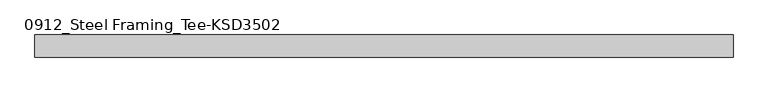
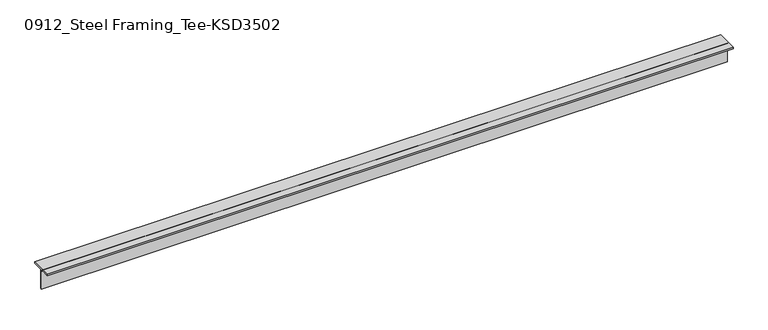
"""IFC4 building model written with IfcOpenShell, lengths in millimetres: member geometry, 0912_Steel Framing_Tee-KSD3502 : H_SB_ASB_CT-150x150x6.5x9."""

from ifc_helpers import new_model, si_unit, point, frame, frame_2d, origin, place, context, project, spatial, polyline, circle_curve, trimmed, segment, composite_curve, outline, extrude, source, transform, mapped, element, save


def member_0912_steel_framing_tee_ksd3502_f996880d(model_context):
    return source(origin(), model_context, "Body", "SweptSolid", [
        extrude(outline(composite_curve([segment(polyline([(-75.0, 75.0), (75.0, 75.0), (75.0, 66.0), (16.25, 66.0)]), True, "CONTINUOUS"), segment(trimmed(circle_curve(frame_2d((16.25, 53.0)), 13.0), [point((16.25, 66.0))], [point((3.25, 53.0))], True, "CARTESIAN"), True, "CONTINUOUS"), segment(polyline([(3.25, 53.0), (3.25, -75.0), (-3.25, -75.0), (-3.25, 53.0)]), True, "CONTINUOUS"), segment(trimmed(circle_curve(frame_2d((-16.25, 53.0)), 13.0), [point((-3.25, 53.0))], [point((-16.25, 66.0))], True, "CARTESIAN"), True, "CONTINUOUS"), segment(polyline([(-16.25, 66.0), (-75.0, 66.0), (-75.0, 75.0)]), True, "CONTINUOUS")], self_intersect=False)), frame((-2315.0, 0.0, 0.0), z_axis=(1.0, 0.0, 0.0), x_axis=(0.0, 1.0, 0.0)), (0.0, 0.0, 1.0), 4728.1),
    ])


if __name__ == "__main__":
    model = new_model("IFC4")
    model_context = context("Model", 3, world=origin())
    ifc_project = project(units=[si_unit("LENGTHUNIT", "METRE", prefix="MILLI")], contexts=[model_context])
    site = spatial("IfcSite", under=ifc_project)
    building = spatial("IfcBuilding", under=site)
    placement = place(None, origin())
    member_0912_steel_framing_tee_ksd3502_shape = member_0912_steel_framing_tee_ksd3502_f996880d(model_context)
    element("IfcMember", 1, ObjectType="0912_Steel Framing_Tee-KSD3502 : H_SB_ASB_CT-150x150x6.5x9", at=placement, inside=building, context=model_context, shape_type="MappedRepresentation", body=[
        mapped(member_0912_steel_framing_tee_ksd3502_shape, transform((0.0, 0.0, 0.0), x_axis=(1.0, 0.0, 0.0), y_axis=(0.0, 1.0, 0.0), z_axis=(0.0, 0.0, 1.0))),
    ])
    save(model, "model.ifc")

# Revit data of these elements
# Type "0912_Steel Framing_Tee-KSD3502 : H_SB_ASB_CT-150x150x6.5x9"
#   H_WM Code_1 = "S01AA003-00001 | Main Steel Structure Fabrication Work | Shelter/Building | Light Steel - Standard (30KG/M>Weight) | Material: (   )"
#   H_WM Code_2 = "S03AA029-00001 | Main Steel Structure Erection Work | Shelter/Building | Light Steel (30KG/M>Weight) | Material: (   )"
#   H_WM Code_3 = "S01AA010-00001 | Main Steel Structure Fabrication Work | Shelter/Building | Steel Painting/Coating | for Non-Fireproofed Steel Surface, Surface Preparation, Primer, Second & Final Coat | Material: (   )"
#   H_Q'ty Cal Type Tag = "SB-Q2"
#   Width = 15.0 cm
#   Web Thickness = 0.65 cm
#   Web Fillet = 1.3 cm
#   Section Area = 23.39 cm²
#   Perimeter = 0.60 m²/m
#   Nominal Weight = 18.40 kgf/m
#   Height = 15.0 cm
#   Flange Thickness = 0.9 cm
#   Centroid Vertical = 7.5 cm
#   Centroid Horizontal = 7.5 cm
#   Length [instance default] = 1.5000 m
#   Structural Material [instance default] = Steel, 45-345
#   Warping Constant = (empty or 0)
#   Torsional Moment of Inertia = 0
#   Section Name Key = ""
#   Plastic Modulus weak axis = 0
#   Plastic Modulus strong axis = 0
#   Moment of Inertia weak axis = 0
#   Moment of Inertia strong axis = 0
#   Elastic Modulus weak axis = 0
#   Elastic Modulus strong axis = 0
#   Bolt Spacing = 0
#   Assembly Code = ""
# Element 1 (IfcMember, "0912_Steel Framing_Tee-KSD3502 : H_SB_ASB_CT-150x150x6.5x9")
#   Structural Material = none
# Materials
#   "Steel, 45-345": class "Metal", colour RGB 189 187 185, transparency 0, Description = "Steel 345 MPa", Cost = 0
